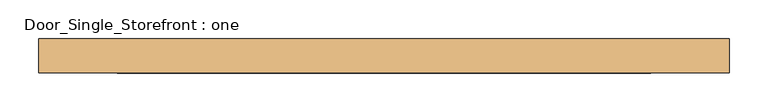
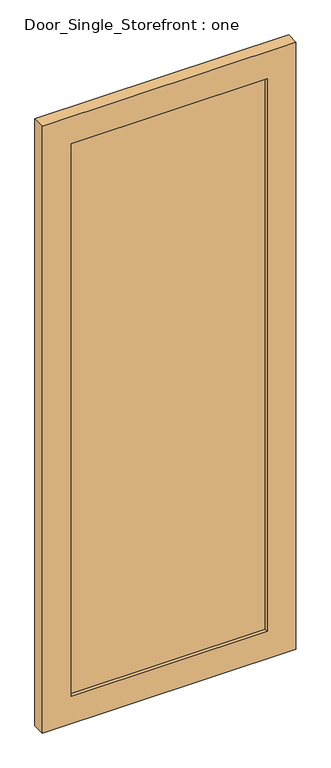
"""IFC4 building model written with IfcOpenShell, lengths in millimetres: door geometry, Door_Single_Storefront : one."""

from ifc_helpers import new_model, si_unit, frame, origin, place, context, project, spatial, polyline, outline, extrude, source, transform, mapped, element, save


def door_single_storefront_one_1e8e98fe(model_context):
    return source(origin(), model_context, "Body", "SweptSolid", [
        extrude(outline(polyline([(345.28125, 19.05), (-345.28125, 19.05), (-345.28125, 38.1), (345.28125, 38.1), (345.28125, 19.05)])), frame((0.0, 0.0, 101.6), z_axis=(0.0, 0.0, 1.0), x_axis=(1.0, 0.0, 0.0)), (0.0, 0.0, 1.0), 2057.4),
        extrude(outline(polyline([(2260.6, -446.88125), (0.0, -446.88125), (0.0, 446.88125), (2260.6, 446.88125), (2260.6, -446.88125)]), holes=[polyline([(101.6, 345.28125), (101.6, -345.28125), (2159.0, -345.28125), (2159.0, 345.28125), (101.6, 345.28125)])]), frame((0.0, 6.35, 0.0), z_axis=(0.0, 1.0, 0.0), x_axis=(0.0, 0.0, 1.0)), (0.0, 0.0, 1.0), 44.45),
    ])


if __name__ == "__main__":
    model = new_model("IFC4")
    model_context = context("Model", 3, world=origin())
    ifc_project = project(units=[si_unit("LENGTHUNIT", "METRE", prefix="MILLI")], contexts=[model_context])
    site = spatial("IfcSite", under=ifc_project)
    building = spatial("IfcBuilding", under=site)
    placement = place(None, origin())
    door_single_storefront_one_shape = door_single_storefront_one_1e8e98fe(model_context)
    element("IfcDoor", 1, ObjectType="Door_Single_Storefront : one", at=placement, inside=building, context=model_context, shape_type="MappedRepresentation", body=[
        mapped(door_single_storefront_one_shape, transform((0.0, 0.0, 0.0), x_axis=(1.0, 0.0, 0.0), y_axis=(0.0, 1.0, 0.0), z_axis=(0.0, 0.0, 1.0))),
    ])
    save(model, "model.ifc")

# Revit data of these elements
# Type "Door_Single_Storefront : one"
#   Type Mark = "27"
#   Analytic Construction = "<None>"
#   Stile_Width = 0' - 4"
#   Door_Thickness = 0' - 1 3/4"
#   Door_Offset = 0' - 2"
#   Glass_Material = Glass
#   Frame_Material = Aluminum
#   Function = (empty or 0)
# Element 1 (IfcDoor, "Door_Single_Storefront : one")
#   Materials on its faces: "Aluminum", "Glass"
# Materials
#   "Glass": class "Glass", colour RGB 0 128 192, transparency 0.75, Description = "Soda Lime Glass", Cost = 0
#   "Aluminum": class "Metal", colour RGB 247 247 247, transparency 0, Description = "Aluminum 6061", Cost = 0
